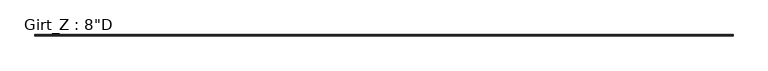
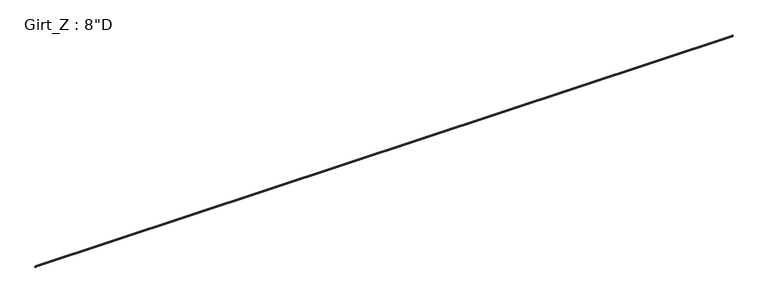
"""IFC4 building model written with IfcOpenShell, lengths in millimetres: beam geometry."""

from ifc_helpers import new_model, si_unit, point, frame, frame_2d, origin, place, context, project, spatial, polyline, circle_curve, trimmed, segment, composite_curve, outline, extrude, source, transform, mapped, element, save


def beam_85d20922(model_context):
    return source(origin(), model_context, "Body", "SweptSolid", [
        extrude(outline(composite_curve([segment(polyline([(-63.5, 101.6), (-3.3734375, 101.6)]), True, "CONTINUOUS"), segment(trimmed(circle_curve(frame_2d((-3.3734375, 96.8375)), 4.7625), [point((-3.3734375, 101.6))], [point((1.3890625, 96.8375))], False, "CARTESIAN"), True, "CONTINUOUS"), segment(polyline([(1.3890625, 96.8375), (1.3890625, -96.8389339)]), True, "CONTINUOUS"), segment(trimmed(circle_curve(frame_2d((3.3748024, -96.8389339)), 1.9857399), [point((1.3890625, -96.8389339))], [point((3.2694106, -98.821875))], True, "CARTESIAN"), True, "CONTINUOUS"), segment(polyline([(3.2694106, -98.821875), (62.204539, -98.821875), (73.6169367, -85.221109), (75.745104, -87.0068534), (63.5, -101.6), (3.3734375, -101.6)]), True, "CONTINUOUS"), segment(trimmed(circle_curve(frame_2d((3.3734375, -96.8375)), 4.7625), [point((3.3734375, -101.6))], [point((-1.3890625, -96.8375))], False, "CARTESIAN"), True, "CONTINUOUS"), segment(polyline([(-1.3890625, -96.8375), (-1.3890625, 96.8381931)]), True, "CONTINUOUS"), segment(trimmed(circle_curve(frame_2d((-3.3741066, 96.8381931)), 1.9850441), [point((-1.3890625, 96.8381931))], [point((-3.3005807, 98.821875))], True, "CARTESIAN"), True, "CONTINUOUS"), segment(polyline([(-3.3005807, 98.821875), (-62.204539, 98.821875), (-73.6169367, 85.221109), (-75.745104, 87.0068534), (-63.5, 101.6)]), True, "CONTINUOUS")], self_intersect=False)), frame((-40618.4447266, 0.0, 0.0), z_axis=(1.0, 0.0, 0.0), x_axis=(0.0, 1.0, 0.0)), (0.0, 0.0, 1.0), 80768.5769531),
    ])


if __name__ == "__main__":
    model = new_model("IFC4")
    model_context = context("Model", 3, world=origin())
    ifc_project = project(units=[si_unit("LENGTHUNIT", "METRE", prefix="MILLI")], contexts=[model_context])
    site = spatial("IfcSite", under=ifc_project)
    building = spatial("IfcBuilding", under=site)
    placement = place(None, origin())
    beam_shape = beam_85d20922(model_context)
    element("IfcBeam", 1, ObjectType="Girt_Z : 8\"D", at=placement, inside=building, context=model_context, shape_type="MappedRepresentation", body=[
        mapped(beam_shape, transform((0.0, 0.0, 0.0), x_axis=(1.0, 0.0, 0.0), y_axis=(0.0, 1.0, 0.0), z_axis=(0.0, 0.0, 1.0))),
    ])
    save(model, "model.ifc")

# Revit data of these elements
# Type "Girt_Z : 8\"D"
#   Web_Thickness = 0' - 0 7/64"
#   Length [instance default] = 10' - 0"
#   Leg_1 = 0' - 2 1/2"
#   Height = 0' - 8"
#   Structural Material [instance default] = none
# Element 1 (IfcBeam, "Girt_Z : 8\"D")
#   Structural Material = Steel
#   Materials on its faces: "Steel"
# Materials
#   "Steel": class "Metal", colour RGB 118 118 114, transparency 0, Description = "Steel, mill finish", Cost = 0
